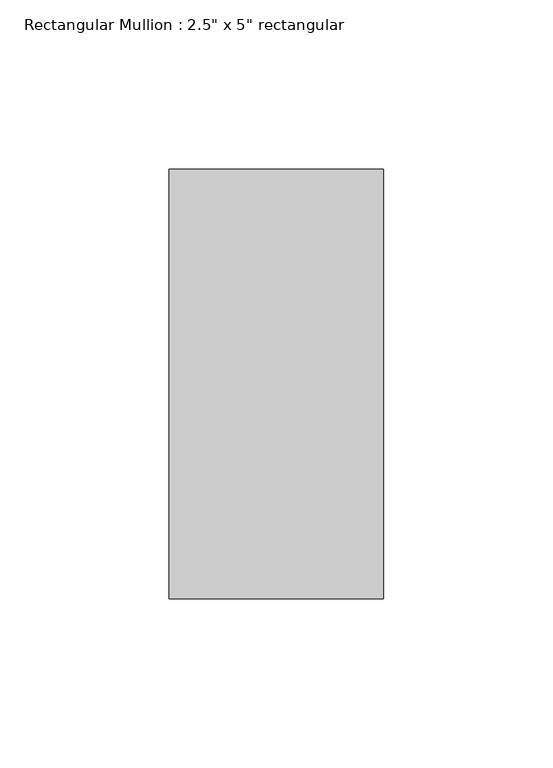
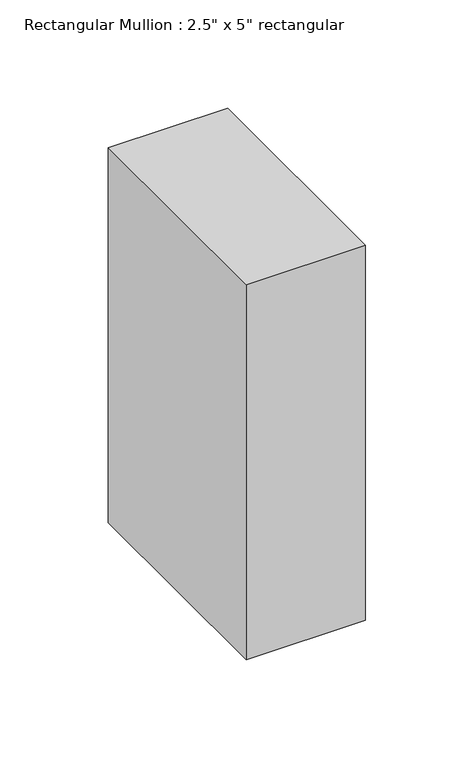
"""IFC4 building model written with IfcOpenShell, lengths in millimetres: member geometry."""

import ifcopenshell
import ifcopenshell.guid

model = None  # the IFC model being written
_history = None  # IfcOwnerHistory: only IFC2X3 demands one
_inside = {}  # id of a spatial element -> (the spatial element, [elements in it])
_under = {}  # id of a project, library or spatial element -> (it, [spatial elements below it])
_declared = {}  # id of a project -> (the project, [libraries it declares])
_typed = {}  # id of a type object -> (the type object, [elements of that type])
_made_of = {}  # id of a material, layer set ... -> (it, [elements and type objects made of it])


def new_model(schema):
    """Start an empty IFC model of exactly this schema.

    Asked for "IFC4X3", IfcOpenShell would pick the latest addendum, in which some entities
    have other attributes; the version numbers below select the first issue.
    IFC2X3 requires an IfcOwnerHistory on every rooted entity: one is made here for all.
    """
    global model, _history
    if schema == "IFC4X3":
        model = ifcopenshell.file(schema_version=(4, 3, 0, 0))
    else:
        model = ifcopenshell.file(schema=schema)
    _inside.clear()
    _under.clear()
    _declared.clear()
    _typed.clear()
    _made_of.clear()
    _history = None
    if model.schema == "IFC2X3":
        org = make("IfcOrganization", Name="unknown")
        user = make(
            "IfcPersonAndOrganization",
            ThePerson=make("IfcPerson", FamilyName="unknown"),
            TheOrganization=org,
        )
        app = make(
            "IfcApplication",
            ApplicationDeveloper=org,
            Version="unknown",
            ApplicationFullName="unknown",
            ApplicationIdentifier="unknown",
        )
        _history = make(
            "IfcOwnerHistory",
            OwningUser=user,
            OwningApplication=app,
            ChangeAction="ADDED",
            CreationDate=0,
        )
    return model


def make(cls, **values):
    """One entity of the class cls with the attributes given. An attribute that is None is left unset."""
    return model.create_entity(
        cls, **{name: value for name, value in values.items() if value is not None}
    )


def rooted(cls, **values):
    """An entity with a GlobalId (a new one), such as an element, a storey or a relation."""
    return make(cls, GlobalId=ifcopenshell.guid.new(), OwnerHistory=_history, **values)


def si_unit(unit_type, name, prefix=None):
    """IfcSIUnit, for example si_unit("LENGTHUNIT", "METRE", prefix="MILLI")."""
    return make("IfcSIUnit", UnitType=unit_type, Prefix=prefix, Name=name)


def assignment(units):
    """IfcUnitAssignment: the units of a project."""
    return None if units is None else make("IfcUnitAssignment", Units=units)


def point(xyz):
    """IfcCartesianPoint."""
    return None if xyz is None else make("IfcCartesianPoint", Coordinates=xyz)


def direction(xyz):
    """IfcDirection."""
    return None if xyz is None else make("IfcDirection", DirectionRatios=xyz)


def frame(location, z_axis=None, x_axis=None):
    """IfcAxis2Placement3D, a coordinate frame: its origin and axes. An axis left out is left unset."""
    return make(
        "IfcAxis2Placement3D",
        Location=point(location),
        Axis=direction(z_axis),
        RefDirection=direction(x_axis),
    )


def origin():
    """The frame at (0, 0, 0) with its axes left unset."""
    return frame((0.0, 0.0, 0.0))


def place(relative_to, where):
    """IfcLocalPlacement: puts the frame where relative to a parent placement (None: the world)."""
    return make(
        "IfcLocalPlacement", PlacementRelTo=relative_to, RelativePlacement=where
    )


def context(
    kind, dimensions, precision=None, world=None, true_north=None, identifier=None
):
    """IfcGeometricRepresentationContext, for example the 3D "Model" context."""
    return make(
        "IfcGeometricRepresentationContext",
        ContextIdentifier=identifier,
        ContextType=kind,
        CoordinateSpaceDimension=dimensions,
        Precision=precision,
        WorldCoordinateSystem=world,
        TrueNorth=true_north,
    )


def project(units=None, contexts=None):
    """IfcProject with its units and contexts."""
    return rooted(
        "IfcProject",
        Name="project",
        RepresentationContexts=contexts,
        UnitsInContext=assignment(units),
    )


def spatial(cls, under=None, at=None, **own):
    """A site, building, storey or space (cls), placed at a placement, below another one or the project."""
    s = rooted(cls, ObjectPlacement=at, **own)
    if under is not None:
        _under.setdefault(under.id(), (under, []))[1].append(s)
    return s


def polyline(points):
    """IfcPolyline through the points."""
    return make("IfcPolyline", Points=[point(p) for p in points])


def outline(outer, holes=None, kind="AREA"):
    """IfcArbitraryClosedProfileDef: a profile drawn as a closed curve; with holes, ...WithVoids."""
    if holes is None:
        return make("IfcArbitraryClosedProfileDef", ProfileType=kind, OuterCurve=outer)
    return make(
        "IfcArbitraryProfileDefWithVoids",
        ProfileType=kind,
        OuterCurve=outer,
        InnerCurves=holes,
    )


def extrude(swept, where, along, depth):
    """IfcExtrudedAreaSolid: the profile swept, set in the frame where, extruded along a direction by depth."""
    return make(
        "IfcExtrudedAreaSolid",
        SweptArea=swept,
        Position=where,
        ExtrudedDirection=direction(along),
        Depth=depth,
    )


def shape(context_of_items, identifier, shape_type, items):
    """IfcShapeRepresentation: the items that make up one representation, for example the "Body"."""
    return make(
        "IfcShapeRepresentation",
        ContextOfItems=context_of_items,
        RepresentationIdentifier=identifier,
        RepresentationType=shape_type,
        Items=items,
    )


def source(mapping_origin, context_of_items, identifier, shape_type, items):
    """IfcRepresentationMap: a shape defined once, which mapped items show again and again."""
    return make(
        "IfcRepresentationMap",
        MappingOrigin=mapping_origin,
        MappedRepresentation=shape(context_of_items, identifier, shape_type, items),
    )


def transform(
    local_origin,
    x_axis=None,
    y_axis=None,
    z_axis=None,
    scale=None,
    scale2=None,
    scale3=None,
    uniform=True,
):
    """IfcCartesianTransformationOperator3D, or its non-uniform kind. x_axis, y_axis, z_axis: its Axis1, 2, 3."""
    if uniform:
        return make(
            "IfcCartesianTransformationOperator3D",
            Axis1=direction(x_axis),
            Axis2=direction(y_axis),
            LocalOrigin=point(local_origin),
            Scale=scale,
            Axis3=direction(z_axis),
        )
    return make(
        "IfcCartesianTransformationOperator3DnonUniform",
        Axis1=direction(x_axis),
        Axis2=direction(y_axis),
        LocalOrigin=point(local_origin),
        Scale=scale,
        Axis3=direction(z_axis),
        Scale2=scale2,
        Scale3=scale3,
    )


def mapped(mapping_source, mapping_target):
    """IfcMappedItem: shows the shape of a source again, moved by a transform."""
    return make(
        "IfcMappedItem", MappingSource=mapping_source, MappingTarget=mapping_target
    )


def made_of(thing, what):
    """Note that an element or type object is made of a material, layer set ...; save() writes the relation."""
    if what is not None:
        _made_of.setdefault(what.id(), (what, []))[1].append(thing)
    return thing


def element(
    cls,
    number,
    at=None,
    inside=None,
    cuts=None,
    type_object=None,
    material=None,
    context=None,
    identifier="Body",
    shape_type=None,
    held_by="IfcProductDefinitionShape",
    body=None,
    shapes=None,
    **own,
):
    """One element of the class cls, such as IfcWall. Its Tag is "e" and its number.

    at: its placement. inside: the storey or other place that contains it. cuts: it is an
    opening in that element (IfcRelVoidsElement). A single representation is given by context,
    identifier, shape_type and body (its items); several are given by shapes. held_by: the class
    of the entity that holds the representations. save() writes the other relations.
    """
    e = rooted(cls, Tag="e%d" % number, ObjectPlacement=at, **own)
    if body is not None:
        shapes = [shape(context, identifier, shape_type, body)]
    if shapes is not None:
        e.Representation = make(held_by, Representations=shapes)
    if inside is not None:
        _inside.setdefault(inside.id(), (inside, []))[1].append(e)
    if cuts is not None:
        rooted(
            "IfcRelVoidsElement", RelatingBuildingElement=cuts, RelatedOpeningElement=e
        )
    if type_object is not None:
        _typed.setdefault(type_object.id(), (type_object, []))[1].append(e)
    return made_of(e, material)


def aggregate(whole, parts):
    """IfcRelAggregates: a whole, such as a stair, and the parts it consists of."""
    return rooted("IfcRelAggregates", RelatingObject=whole, RelatedObjects=parts)


def save(model, path):
    """Write the relations noted so far, then the file.

    IfcRelAggregates (storeys below a building ...), IfcRelContainedInSpatialStructure (elements
    in a storey), IfcRelDefinesByType, IfcRelAssociatesMaterial and IfcRelDeclares: one each for
    every whole, place, type object, material and project.
    """
    for whole, parts in _under.values():
        aggregate(whole, parts)
    for where, things in _inside.values():
        rooted(
            "IfcRelContainedInSpatialStructure",
            RelatedElements=things,
            RelatingStructure=where,
        )
    for kind, things in _typed.values():
        rooted("IfcRelDefinesByType", RelatedObjects=things, RelatingType=kind)
    for what, things in _made_of.values():
        rooted("IfcRelAssociatesMaterial", RelatedObjects=things, RelatingMaterial=what)
    for by, libraries in _declared.values():
        rooted("IfcRelDeclares", RelatingContext=by, RelatedDefinitions=libraries)
    model.write(path)


def member_dd5c6200(model_context):
    return source(origin(), model_context, "Body", "SweptSolid", [
        extrude(outline(polyline([(0.0, 63.5), (0.0, -63.5), (-63.5, -63.5), (-63.5, 63.5), (0.0, 63.5)])), frame((0.0, 0.0, -210.9151287), z_axis=(0.0, 0.0, 1.0), x_axis=(1.0, 0.0, 0.0)), (0.0, 0.0, 1.0), 210.9151287),
    ])


if __name__ == "__main__":
    model = new_model("IFC4")
    model_context = context("Model", 3, world=origin())
    ifc_project = project(units=[si_unit("LENGTHUNIT", "METRE", prefix="MILLI")], contexts=[model_context])
    site = spatial("IfcSite", under=ifc_project)
    building = spatial("IfcBuilding", under=site)
    placement = place(None, origin())
    member_shape = member_dd5c6200(model_context)
    element("IfcMember", 1, ObjectType="Rectangular Mullion : 2.5\" x 5\" rectangular", at=placement, inside=building, context=model_context, shape_type="MappedRepresentation", body=[
        mapped(member_shape, transform((0.0, 0.0, 0.0), x_axis=(1.0, 0.0, 0.0), y_axis=(0.0, 1.0, 0.0), z_axis=(0.0, 0.0, 1.0))),
    ])
    save(model, "model.ifc")

# Revit data of these elements
# Type "Rectangular Mullion : 2.5\" x 5\" rectangular"
#   built-in parameter 1007304 = 0.416667 (stored number, unit not read)
#   built-in parameter 1007301 = 0.104167 (stored number, unit not read)
#   built-in parameter 1007300 = 0.104167 (stored number, unit not read)
# Element 1 (IfcMember, "Rectangular Mullion : 2.5\" x 5\" rectangular")
#   Materials on its faces: "Metal - Aluminum"
# Materials
#   "Metal - Aluminum": class "Metal", colour RGB 140 140 140, transparency 0
